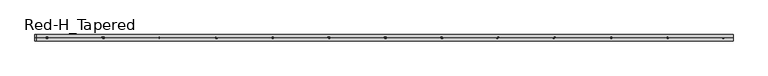
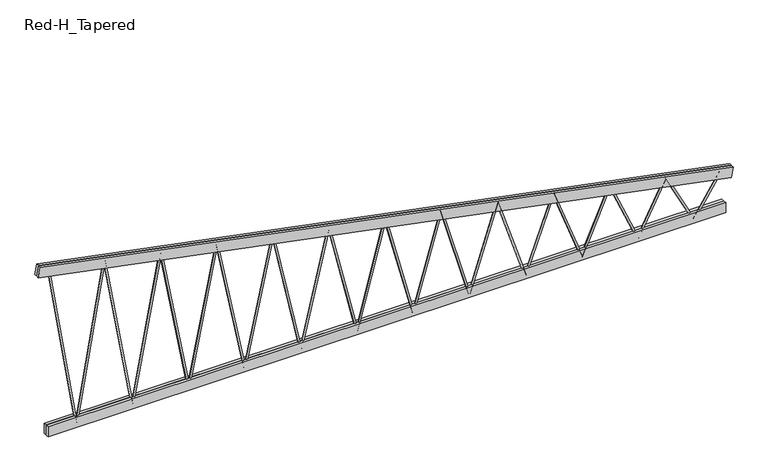
"""IFC4 building model written with IfcOpenShell, lengths in millimetres: beam geometry, Construction_Frames_RedBuilt_Openweb_Red-H_Tapered : Red-H_Tapered."""

from ifc_helpers import new_model, si_unit, point, frame, origin, origin_2d, place, context, project, spatial, polyline, circle_curve, trimmed, segment, composite_curve, outline, extrude, source, transform, mapped, element, save


def red_h_tapered_bd7df729(model_context):
    return source(origin(), model_context, "Body", "SweptSolid", [
        extrude(outline(composite_curve([segment(trimmed(circle_curve(origin_2d(), 12.7), [point((0.0, 12.7))], [point((0.0, -12.7000001))], False, "CARTESIAN"), True, "CONTINUOUS"), segment(trimmed(circle_curve(origin_2d(), 12.7), [point((0.0, -12.7000001))], [point((0.0, 12.7))], False, "CARTESIAN"), True, "CONTINUOUS")], self_intersect=False)), frame((-4144.4333333, 0.0, -367.0101562), z_axis=(-0.1588441891295665, 0.0, 0.9873036633071766), x_axis=(0.0, -1.0, 0.0)), (0.0, 0.0, 1.0), 2371.9260285),
        extrude(outline(composite_curve([segment(trimmed(circle_curve(origin_2d(), 12.7), [point((0.0, -12.7))], [point((0.0, 12.7))], False, "CARTESIAN"), True, "CONTINUOUS"), segment(trimmed(circle_curve(origin_2d(), 12.7), [point((0.0, 12.7))], [point((0.0, -12.7))], False, "CARTESIAN"), True, "CONTINUOUS")], self_intersect=False)), frame((1130.3, 0.0, -367.0101562), z_axis=(-0.2751349261836707, 0.0, 0.9614056232381346), x_axis=(0.0, -1.0, 0.0)), (0.0, 0.0, 1.0), 1369.3887283),
        extrude(outline(composite_curve([segment(trimmed(circle_curve(origin_2d(), 12.7), [point((0.0, 12.7))], [point((0.0, -12.7))], False, "CARTESIAN"), True, "CONTINUOUS"), segment(trimmed(circle_curve(origin_2d(), 12.7), [point((0.0, -12.7))], [point((0.0, 12.7))], False, "CARTESIAN"), True, "CONTINUOUS")], self_intersect=False)), frame((376.7666667, 0.0, -367.0101562), z_axis=(0.2751349261836737, 0.0, 0.9614056232381338), x_axis=(0.0, -1.0, 0.0)), (0.0, 0.0, 1.0), 1369.3887283),
        extrude(outline(composite_curve([segment(trimmed(circle_curve(origin_2d(), 12.7), [point((0.0, -12.7))], [point((0.0, 12.7))], False, "CARTESIAN"), True, "CONTINUOUS"), segment(trimmed(circle_curve(origin_2d(), 12.7), [point((0.0, 12.7))], [point((0.0, -12.7))], False, "CARTESIAN"), True, "CONTINUOUS")], self_intersect=False)), frame((376.7666667, 0.0, -367.0101562), z_axis=(-0.24939195296979247, 0.0, 0.9684026300015469), x_axis=(0.0, -1.0, 0.0)), (0.0, 0.0, 1.0), 1510.7410732),
        extrude(outline(composite_curve([segment(trimmed(circle_curve(origin_2d(), 12.7), [point((0.0, 12.7))], [point((0.0, -12.7))], False, "CARTESIAN"), True, "CONTINUOUS"), segment(trimmed(circle_curve(origin_2d(), 12.7), [point((0.0, -12.7))], [point((0.0, 12.7))], False, "CARTESIAN"), True, "CONTINUOUS")], self_intersect=False)), frame((-376.7666667, 0.0, -367.0101562), z_axis=(0.24939195296976147, 0.0, 0.9684026300015548), x_axis=(0.0, -1.0, 0.0)), (0.0, 0.0, 1.0), 1510.7410732),
        extrude(outline(composite_curve([segment(trimmed(circle_curve(origin_2d(), 12.7), [point((0.0, -12.7))], [point((0.0, 12.7))], False, "CARTESIAN"), True, "CONTINUOUS"), segment(trimmed(circle_curve(origin_2d(), 12.7), [point((0.0, 12.7))], [point((0.0, -12.7))], False, "CARTESIAN"), True, "CONTINUOUS")], self_intersect=False)), frame((-376.7666667, 0.0, -367.0101562), z_axis=(-0.22793117807234023, 0.0, 0.9736772453244222), x_axis=(0.0, -1.0, 0.0)), (0.0, 0.0, 1.0), 1652.9843344),
        extrude(outline(composite_curve([segment(trimmed(circle_curve(origin_2d(), 12.7), [point((0.0, 12.7))], [point((0.0, -12.7))], False, "CARTESIAN"), True, "CONTINUOUS"), segment(trimmed(circle_curve(origin_2d(), 12.7), [point((0.0, -12.7))], [point((0.0, 12.7))], False, "CARTESIAN"), True, "CONTINUOUS")], self_intersect=False)), frame((-1130.3, 0.0, -367.0101562), z_axis=(0.22793117807234073, 0.0, 0.9736772453244221), x_axis=(0.0, -1.0, 0.0)), (0.0, 0.0, 1.0), 1652.9843344),
        extrude(outline(composite_curve([segment(trimmed(circle_curve(origin_2d(), 12.7), [point((0.0, -12.7))], [point((0.0, 12.7))], False, "CARTESIAN"), True, "CONTINUOUS"), segment(trimmed(circle_curve(origin_2d(), 12.7), [point((0.0, 12.7))], [point((0.0, -12.7))], False, "CARTESIAN"), True, "CONTINUOUS")], self_intersect=False)), frame((-1130.3, 0.0, -367.0101562), z_axis=(-0.20979187786626347, 0.0, 0.9777460651832596), x_axis=(0.0, -1.0, 0.0)), (0.0, 0.0, 1.0), 1795.9068316),
        extrude(outline(composite_curve([segment(trimmed(circle_curve(origin_2d(), 12.7), [point((0.0, -12.7000001))], [point((0.0, 12.7))], False, "CARTESIAN"), True, "CONTINUOUS"), segment(trimmed(circle_curve(origin_2d(), 12.7), [point((0.0, 12.7))], [point((0.0, -12.7000001))], False, "CARTESIAN"), True, "CONTINUOUS")], self_intersect=False)), frame((-1883.8333333, 0.0, -367.0101562), z_axis=(0.20979187786626646, 0.0, 0.9777460651832589), x_axis=(0.0, -1.0, 0.0)), (0.0, 0.0, 1.0), 1795.9068316),
        extrude(outline(composite_curve([segment(trimmed(circle_curve(origin_2d(), 12.7), [point((0.0, 12.6999999))], [point((0.0, -12.7))], False, "CARTESIAN"), True, "CONTINUOUS"), segment(trimmed(circle_curve(origin_2d(), 12.7), [point((0.0, -12.7))], [point((0.0, 12.6999999))], False, "CARTESIAN"), True, "CONTINUOUS")], self_intersect=False)), frame((-1883.8333333, 0.0, -367.0101562), z_axis=(-0.19427387255590262, 0.0, 0.9809473290865993), x_axis=(0.0, -1.0, 0.0)), (0.0, 0.0, 1.0), 1939.3584001),
        extrude(outline(composite_curve([segment(trimmed(circle_curve(origin_2d(), 12.7), [point((0.0, -12.6999999))], [point((0.0, 12.7))], False, "CARTESIAN"), True, "CONTINUOUS"), segment(trimmed(circle_curve(origin_2d(), 12.7), [point((0.0, 12.7))], [point((0.0, -12.6999999))], False, "CARTESIAN"), True, "CONTINUOUS")], self_intersect=False)), frame((-2637.3666667, 0.0, -367.0101562), z_axis=(0.19427387255590164, 0.0, 0.9809473290865995), x_axis=(0.0, -1.0, 0.0)), (0.0, 0.0, 1.0), 1939.3584001),
        extrude(outline(composite_curve([segment(trimmed(circle_curve(origin_2d(), 12.7), [point((0.0, 12.7000001))], [point((0.0, -12.7))], False, "CARTESIAN"), True, "CONTINUOUS"), segment(trimmed(circle_curve(origin_2d(), 12.7), [point((0.0, -12.7))], [point((0.0, 12.7000001))], False, "CARTESIAN"), True, "CONTINUOUS")], self_intersect=False)), frame((-2637.3666667, 0.0, -367.0101562), z_axis=(-0.180856992463189, 0.0, 0.983509404264733), x_axis=(0.0, -1.0, 0.0)), (0.0, 0.0, 1.0), 2083.2297471),
        extrude(outline(composite_curve([segment(trimmed(circle_curve(origin_2d(), 12.7), [point((0.0, -12.7))], [point((0.0, 12.7))], False, "CARTESIAN"), True, "CONTINUOUS"), segment(trimmed(circle_curve(origin_2d(), 12.7), [point((0.0, 12.7))], [point((0.0, -12.7))], False, "CARTESIAN"), True, "CONTINUOUS")], self_intersect=False)), frame((-3390.9, 0.0, -367.0101562), z_axis=(0.18085699246319326, 0.0, 0.9835094042647322), x_axis=(0.0, -1.0, 0.0)), (0.0, 0.0, 1.0), 2083.2297471),
        extrude(outline(composite_curve([segment(trimmed(circle_curve(origin_2d(), 12.7), [point((0.0, 12.7))], [point((0.0, -12.7))], False, "CARTESIAN"), True, "CONTINUOUS"), segment(trimmed(circle_curve(origin_2d(), 12.7), [point((0.0, -12.7))], [point((0.0, 12.7))], False, "CARTESIAN"), True, "CONTINUOUS")], self_intersect=False)), frame((-3390.9, 0.0, -367.0101562), z_axis=(-0.16914787634304293, 0.0, 0.9855906837671705), x_axis=(0.0, -1.0, 0.0)), (0.0, 0.0, 1.0), 2227.4395329),
        extrude(outline(composite_curve([segment(trimmed(circle_curve(origin_2d(), 12.7), [point((0.0, -12.7))], [point((0.0, 12.7))], False, "CARTESIAN"), True, "CONTINUOUS"), segment(trimmed(circle_curve(origin_2d(), 12.7), [point((0.0, 12.7))], [point((0.0, -12.7))], False, "CARTESIAN"), True, "CONTINUOUS")], self_intersect=False)), frame((-4144.4333333, 0.0, -367.0101562), z_axis=(0.16914787634304163, 0.0, 0.9855906837671707), x_axis=(0.0, -1.0, 0.0)), (0.0, 0.0, 1.0), 2227.4395329),
        extrude(outline(composite_curve([segment(trimmed(circle_curve(origin_2d(), 12.7), [point((0.0, 12.7))], [point((0.0, -12.7))], False, "CARTESIAN"), True, "CONTINUOUS"), segment(trimmed(circle_curve(origin_2d(), 12.7), [point((0.0, -12.7))], [point((0.0, 12.7))], False, "CARTESIAN"), True, "CONTINUOUS")], self_intersect=False)), frame((4144.4333333, 0.0, -367.0101562), z_axis=(0.5419881538462402, 0.0, 0.8403861261886374), x_axis=(0.0, -1.0, 0.0)), (0.0, 0.0, 1.0), 695.156645),
        extrude(outline(composite_curve([segment(trimmed(circle_curve(origin_2d(), 12.7), [point((0.0, -12.7))], [point((0.0, 12.7))], False, "CARTESIAN"), True, "CONTINUOUS"), segment(trimmed(circle_curve(origin_2d(), 12.7), [point((0.0, 12.7))], [point((0.0, -12.7))], False, "CARTESIAN"), True, "CONTINUOUS")], self_intersect=False)), frame((4144.4333333, 0.0, -367.0101562), z_axis=(-0.4583046838689422, 0.0, 0.8887951489200361), x_axis=(0.0, -1.0, 0.0)), (0.0, 0.0, 1.0), 822.0877506),
        extrude(outline(composite_curve([segment(trimmed(circle_curve(origin_2d(), 12.7), [point((0.0, 12.7))], [point((0.0, -12.7))], False, "CARTESIAN"), True, "CONTINUOUS"), segment(trimmed(circle_curve(origin_2d(), 12.7), [point((0.0, -12.7))], [point((0.0, 12.7))], False, "CARTESIAN"), True, "CONTINUOUS")], self_intersect=False)), frame((3390.9, 0.0, -367.0101562), z_axis=(0.45830468386894385, 0.0, 0.8887951489200352), x_axis=(0.0, -1.0, 0.0)), (0.0, 0.0, 1.0), 822.0877506),
        extrude(outline(composite_curve([segment(trimmed(circle_curve(origin_2d(), 12.7), [point((0.0, -12.7))], [point((0.0, 12.7))], False, "CARTESIAN"), True, "CONTINUOUS"), segment(trimmed(circle_curve(origin_2d(), 12.7), [point((0.0, 12.7))], [point((0.0, -12.7))], False, "CARTESIAN"), True, "CONTINUOUS")], self_intersect=False)), frame((3390.9, 0.0, -367.0101562), z_axis=(-0.3946727935442272, 0.0, 0.91882173789914), x_axis=(0.0, -1.0, 0.0)), (0.0, 0.0, 1.0), 954.6304504),
        extrude(outline(composite_curve([segment(trimmed(circle_curve(origin_2d(), 12.7), [point((0.0, 12.6999999))], [point((0.0, -12.7))], False, "CARTESIAN"), True, "CONTINUOUS"), segment(trimmed(circle_curve(origin_2d(), 12.7), [point((0.0, -12.7))], [point((0.0, 12.6999999))], False, "CARTESIAN"), True, "CONTINUOUS")], self_intersect=False)), frame((2637.3666667, 0.0, -367.0101562), z_axis=(0.3946727935442274, 0.0, 0.9188217378991399), x_axis=(0.0, -1.0, 0.0)), (0.0, 0.0, 1.0), 954.6304504),
        extrude(outline(composite_curve([segment(trimmed(circle_curve(origin_2d(), 12.7), [point((0.0, -12.7))], [point((0.0, 12.7))], False, "CARTESIAN"), True, "CONTINUOUS"), segment(trimmed(circle_curve(origin_2d(), 12.7), [point((0.0, 12.7))], [point((0.0, -12.7))], False, "CARTESIAN"), True, "CONTINUOUS")], self_intersect=False)), frame((2637.3666667, 0.0, -367.0101562), z_axis=(-0.3454226808968656, 0.0, 0.9384472129651311), x_axis=(0.0, -1.0, 0.0)), (0.0, 0.0, 1.0), 1090.7409603),
        extrude(outline(composite_curve([segment(trimmed(circle_curve(origin_2d(), 12.7), [point((0.0, 12.7))], [point((0.0, -12.7))], False, "CARTESIAN"), True, "CONTINUOUS"), segment(trimmed(circle_curve(origin_2d(), 12.7), [point((0.0, -12.7))], [point((0.0, 12.7))], False, "CARTESIAN"), True, "CONTINUOUS")], self_intersect=False)), frame((1883.8333333, 0.0, -367.0101562), z_axis=(0.345422680896868, 0.0, 0.9384472129651302), x_axis=(0.0, -1.0, 0.0)), (0.0, 0.0, 1.0), 1090.7409603),
        extrude(outline(composite_curve([segment(trimmed(circle_curve(origin_2d(), 12.7), [point((0.0, -12.7))], [point((0.0, 12.7))], False, "CARTESIAN"), True, "CONTINUOUS"), segment(trimmed(circle_curve(origin_2d(), 12.7), [point((0.0, 12.7))], [point((0.0, -12.7))], False, "CARTESIAN"), True, "CONTINUOUS")], self_intersect=False)), frame((1883.8333333, 0.0, -367.0101562), z_axis=(-0.30650507327676635, 0.0, 0.9518690246329082), x_axis=(0.0, -1.0, 0.0)), (0.0, 0.0, 1.0), 1229.2346833),
        extrude(outline(composite_curve([segment(trimmed(circle_curve(origin_2d(), 12.7), [point((0.0, 12.7))], [point((0.0, -12.7))], False, "CARTESIAN"), True, "CONTINUOUS"), segment(trimmed(circle_curve(origin_2d(), 12.7), [point((0.0, -12.7))], [point((0.0, 12.7))], False, "CARTESIAN"), True, "CONTINUOUS")], self_intersect=False)), frame((1130.3, 0.0, -367.0101562), z_axis=(0.3065050732767705, 0.0, 0.951869024632907), x_axis=(0.0, -1.0, 0.0)), (0.0, 0.0, 1.0), 1229.2346833),
        extrude(outline(polyline([(-4546.6, -41.275), (-4546.6, -3.175), (4546.6, -3.175), (4546.6, -41.275), (-4546.6, -41.275)])), frame((0.0, 0.0, -386.0601562), z_axis=(0.0, 0.0, 1.0), x_axis=(1.0, 0.0, 0.0)), (0.0, 0.0, 1.0), 139.7),
        extrude(outline(polyline([(-4546.6, 3.175), (-4546.6, 41.275), (4546.6, 41.275), (4546.6, 3.175), (-4546.6, 3.175)])), frame((0.0, 0.0, -386.0601562), z_axis=(0.0, 0.0, 1.0), x_axis=(1.0, 0.0, 0.0)), (0.0, 0.0, 1.0), 139.7),
        extrude(outline(polyline([(0.0, -38.1), (0.0, 0.0), (9474.5745234, 0.0), (9474.5745234, -38.1), (0.0, -38.1)])), frame((-4675.1651539, -3.175, 1915.2669782), z_axis=(0.19302186029333465, 0.0, 0.981194456491118), x_axis=(0.981194456491118, 0.0, -0.19302186029333465)), (0.0, 0.0, 1.0), 139.7),
        extrude(outline(polyline([(0.0, -38.1), (0.0, 0.0), (9474.5745234, 0.0), (9474.5745234, -38.1), (0.0, -38.1)])), frame((-4675.1651539, 41.275, 1915.2669782), z_axis=(0.19302186029333465, 0.0, 0.981194456491118), x_axis=(0.981194456491118, 0.0, -0.19302186029333465)), (0.0, 0.0, 1.0), 139.7),
    ])


if __name__ == "__main__":
    model = new_model("IFC4")
    model_context = context("Model", 3, world=origin())
    ifc_project = project(units=[si_unit("LENGTHUNIT", "METRE", prefix="MILLI")], contexts=[model_context])
    site = spatial("IfcSite", under=ifc_project)
    building = spatial("IfcBuilding", under=site)
    placement = place(None, origin())
    red_h_tapered_shape = red_h_tapered_bd7df729(model_context)
    element("IfcBeam", 1, ObjectType="Construction_Frames_RedBuilt_Openweb_Red-H_Tapered : Red-H_Tapered", at=placement, inside=building, context=model_context, shape_type="MappedRepresentation", body=[
        mapped(red_h_tapered_shape, transform((0.0, 0.0, 0.0), x_axis=(1.0, 0.0, 0.0), y_axis=(0.0, 1.0, 0.0), z_axis=(0.0, 0.0, 1.0))),
    ])
    save(model, "model.ifc")

# Revit data of these elements
# Type "Construction_Frames_RedBuilt_Openweb_Red-H_Tapered : Red-H_Tapered"
#   Youtube clip = ""
#   Weight Net (Kg) = "0"
#   Webs = "Up to 2\" diameter tubular steel"
#   Uniformat II Description = ""
#   Uniformat II Code = ""
#   Uniclass 2015 Name = "Softwood trusses"
#   Uniclass 2015 Code = "Pr_20_85_90_81"
#   Uniclass 2.0 Description = "Structural Framing Systems"
#   Uniclass 2.0 Code = "SS-15-10-75"
#   Uniclass 1.4 Description = "Trusses"
#   Uniclass 1.4 Code = "L3523"
#   UNSPSC Code = "30103606"
#   Technical description = "http://www.redbuilt.com/reference/literature-and-other-resources"
#   Region South America = "None"
#   Region Oceania = "None"
#   Region North America = "US"
#   Region Middle East = "None"
#   Region Europe = "None"
#   Region Asia = "None"
#   Region Antarctica = "None"
#   Region Africa = "None"
#   QR code = "http://bimobject.com/redbuilt/product/redbuilt-0003"
#   Product url = "http://www.redbuilt.com/products/default.aspx?id=2"
#   Product group = "Wood Trusses"
#   Product family = "Construction"
#   Product data url = "https://bimobject.com/redbuilt/product/redbuilt-0003"
#   Product certification = ""
#   Product SKU = "redbuilt-0003"
#   Product Page URL = "http://www.redbuilt.com/commercial-systems/red-m-red-h-open-web-trusses"
#   Product Guid = "2c5793f2-6ffb-4665-b825-cf90c048e711"
#   Product Documentation Link = "http://www.redbuilt.com/documents/OW_Guide_2017_07_LowRes_wLinks.pdf"
#   OmniClass Description = "Wood Trusses"
#   OmniClass Code = "23-13 35 19 13 17"
#   NBS Reference Description = ""
#   NBS Reference Code = ""
#   Material secondary = "Steel"
#   Material main = "Wood"
#   Masterformat 2014 Description = "Metal-Web Wood Joists"
#   Masterformat 2014 Code = "06 17 36"
#   Manufacturer name = "RedBuilt"
#   Manufacturer country = "United States"
#   Installation instructions = "http://www.redbuilt.com/documents/Installation_Sheets_Open-Web.pdf"
#   IFC Classification = ""
#   EAN code = ""
#   Design country = "United States"
#   Product Information = "http://redbuilt.com/products/default.aspx?id=2"
#   Model = "Red-H-Tapered"
#   Manufacturer URL = "http://redbuilt.com/"
#   Manufacturer = "RedBuilt™"
#   Description = "Open Web Truss"
#   Date of publishing = "8/17/2010"
#   Contact us = "http://redbuilt.com/contact/"
#   Chords = "Double 1½\" x 5½\" MSR lumber"
#   COBIe Type Category = ""
#   Brand url = "http://www.redbuilt.com"
#   BIMobject main category code = "construction"
#   BIMobject main category = "Construction"
#   BIMobject category code = "construction-frames-trusses"
#   BIMobject category = "Frames & Trusses"
#   Web Radius = 0' - 0 1/2"
#   Web Layout Offset Start [instance default] = 0' - 5"
#   Web Layout Offset End [instance default] = 0' - 5"
#   Web Diameter = 0' - 1"
#   TotalLength [instance default] = 20' - 0"
#   Span Minimum = 4' - 0"
#   Span Maximum = 70' - 0"
#   Span Limit [instance default] = 20' - 0"
#   Nominal width = 0' - 0"
#   Nominal height = 0' - 0"
#   Inner Depth Top [instance default] = 0' - 2.76372"
#   Depth Start [instance default] = 6' - 0"
#   Top Chord Length [instance default] = 20' - 1.19701"
#   TC Extension Start Aux [instance default] = 0' - 0"
#   TC Extension End Aux [instance default] = 0' - 0"
#   T-B Chord Length Difference L [instance default] = 0' - 4"
#   T-B Chord Length Difference [instance default] = 0' - 4"
#   Height 2 [instance default] = 6' - 0"
#   Depth Minimum at Wall = 2' - 0"
#   Depth Maximum at Wall = 6' - 0"
#   Depth Lower End [instance default] = 2' - 0"
#   Depth Higher End [instance default] = 6' - 0"
#   Depth End [instance default] = 2' - 0"
#   Depth 2 [instance default] = 2' - 0"
#   Chord Width = 0' - 3 1/4"
#   Chord Thickness = 0' - 1 1/2"
#   Chord Depth = 0' - 5 1/2"
#   Offset Start [instance default] = 0' - 0"
#   TC Extension Start [instance default] = 0' - 0"
#   End Panel = 0' - 5"
#   Offset End [instance default] = 0' - 0"
#   TC Extension End [instance default] = 0' - 0"
#   Length [instance default] = 20' - 0"
#   Angle [instance default] = 5.71059°
#   Span Limit Warning [instance default] = no
#   Edition number = 1
#   Top Bearing Start [instance default] = yes
#   Top Bearing End [instance default] = yes
#   Bottom Bearing Start [instance default] = no
#   Bottom Bearing End [instance default] = no
#   8 Panels [instance default] = yes
#   16 Panels [instance default] = no
#   12 Panels [instance default] = no
#   Web Material = RedBuilt-Steel, Galvanized
#   Clip Material = RedBuilt-Steel, Galvanized
#   Chords Material = RedBuilt-MSR
#   URL = ""
#   Assembly Code = ""
# Element 1 (IfcBeam, "Construction_Frames_RedBuilt_Openweb_Red-H_Tapered : Red-H_Tapered")
#   TotalLength = 30' - 6"
#   Span Limit = 30' - 6"
#   Inner Depth Top = 0' - 2.80271"
#   Top Chord Length = 31' - 1.01475"
#   Depth 2 = 6' - 0"
#   Angle = 11.1292°
#   8 Panels = no
#   12 Panels = yes
#   Materials on its faces: "RedBuilt-Steel, Galvanized", "RedBuilt-MSR"
# Materials
#   "RedBuilt-Steel, Galvanized": class "Metal", colour RGB 164 172 176, transparency 0, Manufacturer = "RedBuilt. LLC", Comments = "Openweb Metal Web", URL = "http://www.redbuilt.com/", Description = "Galvanized steel", Cost = 0
#   "RedBuilt-MSR": class "Wood", colour RGB 213 182 136, transparency 0, Manufacturer = "RedBuilt, LLC", URL = "http://www.redbuilt.com/", Cost = 0
